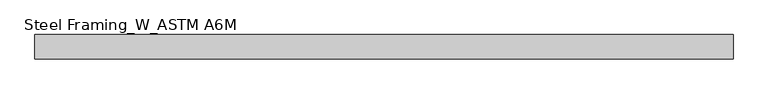
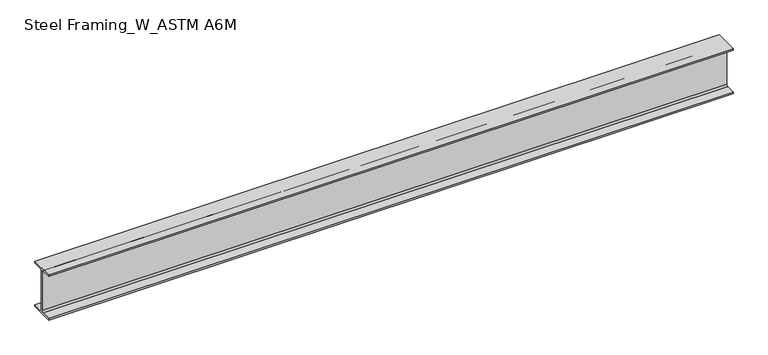
"""IFC4 building model written with IfcOpenShell, lengths in millimetres: beam geometry, Steel Framing_W_ASTM A6M : H_SB_AR_S02_W200x22.5_J1."""

from ifc_helpers import new_model, si_unit, point, frame, frame_2d, origin, place, context, project, spatial, polyline, circle_curve, trimmed, segment, composite_curve, outline, extrude, source, transform, mapped, element, save


def steel_framing_w_astm_a6m_97080517(model_context):
    return source(origin(), model_context, "Body", "SweptSolid", [
        extrude(outline(composite_curve([segment(polyline([(51.0, -95.0), (51.0, -103.0), (-51.0, -103.0), (-51.0, -95.0), (-10.71, -95.0)]), True, "CONTINUOUS"), segment(trimmed(circle_curve(frame_2d((-10.71, -87.4)), 7.6), [point((-10.71, -95.0))], [point((-3.11, -87.4))], True, "CARTESIAN"), True, "CONTINUOUS"), segment(polyline([(-3.11, -87.4), (-3.11, 87.4)]), True, "CONTINUOUS"), segment(trimmed(circle_curve(frame_2d((-10.71, 87.4)), 7.6), [point((-3.11, 87.4))], [point((-10.71, 95.0))], True, "CARTESIAN"), True, "CONTINUOUS"), segment(polyline([(-10.71, 95.0), (-51.0, 95.0), (-51.0, 103.0), (51.0, 103.0), (51.0, 95.0), (10.71, 95.0)]), True, "CONTINUOUS"), segment(trimmed(circle_curve(frame_2d((10.71, 87.4)), 7.6), [point((10.71, 95.0))], [point((3.11, 87.4))], True, "CARTESIAN"), True, "CONTINUOUS"), segment(polyline([(3.11, 87.4), (3.11, -87.4)]), True, "CONTINUOUS"), segment(trimmed(circle_curve(frame_2d((10.71, -87.4)), 7.6), [point((3.11, -87.4))], [point((10.71, -95.0))], True, "CARTESIAN"), True, "CONTINUOUS"), segment(polyline([(10.71, -95.0), (51.0, -95.0)]), True, "CONTINUOUS")], self_intersect=False)), frame((-1470.3, 0.0, 0.0), z_axis=(1.0, 0.0, 0.0), x_axis=(0.0, 1.0, 0.0)), (0.0, 0.0, 1.0), 2940.6),
    ])


if __name__ == "__main__":
    model = new_model("IFC4")
    model_context = context("Model", 3, world=origin())
    ifc_project = project(units=[si_unit("LENGTHUNIT", "METRE", prefix="MILLI")], contexts=[model_context])
    site = spatial("IfcSite", under=ifc_project)
    building = spatial("IfcBuilding", under=site)
    placement = place(None, origin())
    steel_framing_w_astm_a6m_shape = steel_framing_w_astm_a6m_97080517(model_context)
    element("IfcBeam", 1, ObjectType="Steel Framing_W_ASTM A6M : H_SB_AR_S02_W200x22.5_J1", at=placement, inside=building, context=model_context, shape_type="MappedRepresentation", body=[
        mapped(steel_framing_w_astm_a6m_shape, transform((0.0, 0.0, 0.0), x_axis=(1.0, 0.0, 0.0), y_axis=(0.0, 1.0, 0.0), z_axis=(0.0, 0.0, 1.0))),
    ])
    save(model, "model.ifc")

# Revit data of these elements
# Type "Steel Framing_W_ASTM A6M : H_SB_AR_S02_W200x22.5_J1"
#   Section Name Key = "W8x15"
#   Width = 10.2 cm
#   Web Thickness = 0.622 cm
#   Web Fillet = 0.76 cm
#   Warping Constant = 13900.0 cm⁶
#   Torsional Moment of Inertia = 5.70 cm⁴
#   Section Area = 28.6 cm²
#   Plastic Modulus weak axis = 43.8 cm³
#   Plastic Modulus strong axis = 223.0 cm³
#   Perimeter = 0.795 m²/m
#   Nominal Weight = 22.50 kgf/m
#   Moment of Inertia weak axis = 142.00 cm⁴
#   Moment of Inertia strong axis = 2000.00 cm⁴
#   Height = 20.6 cm
#   Flange Thickness = 0.8 cm
#   Elastic Modulus weak axis = 27.9 cm³
#   Elastic Modulus strong axis = 193.0 cm³
#   Centroid Vertical = 10.3 cm
#   Centroid Horizontal = 5.1 cm
#   Length [instance default] = 1500 mm
#   Structural Material [instance default] = Steel, 45-345
#   Bolt Spacing = 0
#   Assembly Code = ""
# Element 1 (IfcBeam, "Steel Framing_W_ASTM A6M : H_SB_AR_S02_W200x22.5_J1")
#   Materials on its faces: "Steel, 45-345"
# Materials
#   "Steel, 45-345": class "Metal", colour RGB 189 187 185, transparency 0, Description = "Steel 345 MPa", Cost = 0
